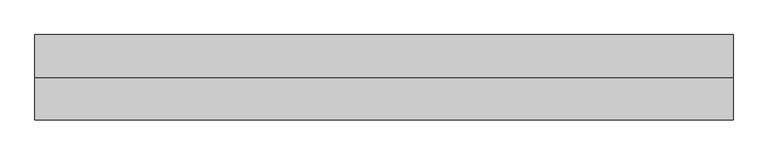
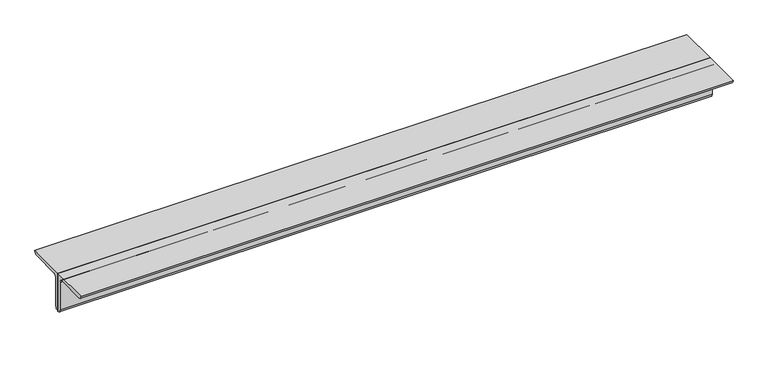
"""IFC4 building model written with IfcOpenShell, lengths in millimetres: member geometry, 0123_Steel Framing_2Ls-KSD3502 : H_SB_AR_S04_2Ls-130x130x12_VBR1."""

from ifc_helpers import new_model, si_unit, point, frame, frame_2d, origin, place, context, project, spatial, polyline, circle_curve, trimmed, segment, composite_curve, outline, extrude, source, transform, mapped, element, save


def member_a6789790(model_context):
    return source(origin(), model_context, "Body", "SweptSolid", [
        extrude(outline(composite_curve([segment(polyline([(0.0, 36.4), (130.0, 36.4)]), True, "CONTINUOUS"), segment(trimmed(circle_curve(frame_2d((118.0, 36.4)), 12.0), [point((130.0, 36.4))], [point((118.0, 24.4))], False, "CARTESIAN"), True, "CONTINUOUS"), segment(polyline([(118.0, 24.4), (24.0, 24.4)]), True, "CONTINUOUS"), segment(trimmed(circle_curve(frame_2d((24.0, 12.4)), 12.0), [point((24.0, 24.4))], [point((12.0, 12.4))], True, "CARTESIAN"), True, "CONTINUOUS"), segment(polyline([(12.0, 12.4), (12.0, -81.6)]), True, "CONTINUOUS"), segment(trimmed(circle_curve(frame_2d((0.0, -81.6)), 12.0), [point((12.0, -81.6))], [point((0.0, -93.6))], False, "CARTESIAN"), True, "CONTINUOUS"), segment(polyline([(0.0, -93.6), (0.0, 36.4)]), True, "CONTINUOUS")], self_intersect=False)), frame((-1023.6979116, 0.0, 0.0), z_axis=(1.0, 0.0, 0.0), x_axis=(0.0, 1.0, 0.0)), (0.0, 0.0, 1.0), 2122.0741046),
        extrude(outline(composite_curve([segment(polyline([(0.0, 36.4), (0.0, -93.6)]), True, "CONTINUOUS"), segment(trimmed(circle_curve(frame_2d((0.0, -81.6)), 12.0), [point((0.0, -93.6))], [point((-12.0, -81.6))], False, "CARTESIAN"), True, "CONTINUOUS"), segment(polyline([(-12.0, -81.6), (-12.0, 12.4)]), True, "CONTINUOUS"), segment(trimmed(circle_curve(frame_2d((-24.0, 12.4)), 12.0), [point((-12.0, 12.4))], [point((-24.0, 24.4))], True, "CARTESIAN"), True, "CONTINUOUS"), segment(polyline([(-24.0, 24.4), (-118.0, 24.4)]), True, "CONTINUOUS"), segment(trimmed(circle_curve(frame_2d((-118.0, 36.4)), 12.0), [point((-118.0, 24.4))], [point((-130.0, 36.4))], False, "CARTESIAN"), True, "CONTINUOUS"), segment(polyline([(-130.0, 36.4), (0.0, 36.4)]), True, "CONTINUOUS")], self_intersect=False)), frame((-1023.6979116, 0.0, 0.0), z_axis=(1.0, 0.0, 0.0), x_axis=(0.0, 1.0, 0.0)), (0.0, 0.0, 1.0), 2122.0741046),
    ])


if __name__ == "__main__":
    model = new_model("IFC4")
    model_context = context("Model", 3, world=origin())
    ifc_project = project(units=[si_unit("LENGTHUNIT", "METRE", prefix="MILLI")], contexts=[model_context])
    site = spatial("IfcSite", under=ifc_project)
    building = spatial("IfcBuilding", under=site)
    placement = place(None, origin())
    member_shape = member_a6789790(model_context)
    element("IfcMember", 1, ObjectType="0123_Steel Framing_2Ls-KSD3502 : H_SB_AR_S04_2Ls-130x130x12_VBR1", at=placement, inside=building, context=model_context, shape_type="MappedRepresentation", body=[
        mapped(member_shape, transform((0.0, 0.0, 0.0), x_axis=(1.0, 0.0, 0.0), y_axis=(0.0, 1.0, 0.0), z_axis=(0.0, 0.0, 1.0))),
    ])
    save(model, "model.ifc")

# Revit data of these elements
# Type "0123_Steel Framing_2Ls-KSD3502 : H_SB_AR_S04_2Ls-130x130x12_VBR1"
#   Assembly Code = "B10"
#   Legs = "SLBB"
#   W = 8.97
#   Perimeter = 1.04 m²/m
#   Nominal Weight = 46.80 kgf/m
#   Length [instance default] = 1000 mm
#   Space = 0 mm
#   b = 130 mm
#   d = 130 mm
#   t = 12 mm
#   y = 36.4 mm
#   A = 0.005952 m²
#   Structural Material [instance default] = Steel ASTM A36
# Element 1 (IfcMember, "0123_Steel Framing_2Ls-KSD3502 : H_SB_AR_S04_2Ls-130x130x12_VBR1")
#   Structural Material = Steel, 45-345
#   Materials on its faces: "Steel, 45-345"
# Materials
#   "Steel ASTM A36": class "Metal", colour RGB 199 199 199, transparency 0, Description = "Structural steel, ASTM A36 Grade B, mill finish", Cost = 0
#   "Steel, 45-345": class "Metal", colour RGB 189 187 185, transparency 0, Description = "Steel 345 MPa", Cost = 0
